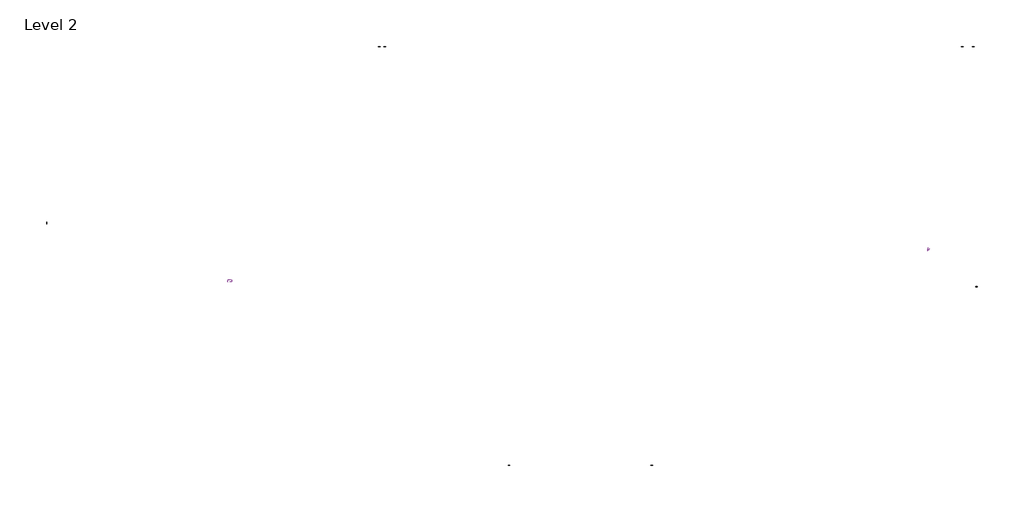
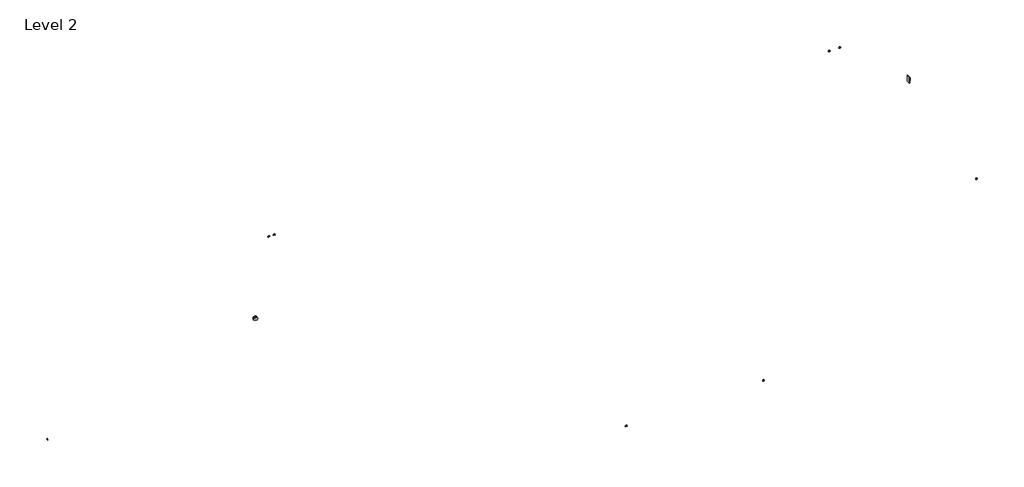
# One storey: 10 proxies.
"""IFC4 building model written with IfcOpenShell, lengths in millimetres."""

import ifcopenshell
import ifcopenshell.guid

model = None  # the IFC model being written
_history = None  # IfcOwnerHistory: only IFC2X3 demands one
_inside = {}  # id of a spatial element -> (the spatial element, [elements in it])
_under = {}  # id of a project, library or spatial element -> (it, [spatial elements below it])
_declared = {}  # id of a project -> (the project, [libraries it declares])
_typed = {}  # id of a type object -> (the type object, [elements of that type])
_made_of = {}  # id of a material, layer set ... -> (it, [elements and type objects made of it])


def new_model(schema):
    """Start an empty IFC model of exactly this schema.

    Asked for "IFC4X3", IfcOpenShell would pick the latest addendum, in which some entities
    have other attributes; the version numbers below select the first issue.
    IFC2X3 requires an IfcOwnerHistory on every rooted entity: one is made here for all.
    """
    global model, _history
    if schema == "IFC4X3":
        model = ifcopenshell.file(schema_version=(4, 3, 0, 0))
    else:
        model = ifcopenshell.file(schema=schema)
    _inside.clear()
    _under.clear()
    _declared.clear()
    _typed.clear()
    _made_of.clear()
    _history = None
    if model.schema == "IFC2X3":
        org = make("IfcOrganization", Name="unknown")
        user = make(
            "IfcPersonAndOrganization",
            ThePerson=make("IfcPerson", FamilyName="unknown"),
            TheOrganization=org,
        )
        app = make(
            "IfcApplication",
            ApplicationDeveloper=org,
            Version="unknown",
            ApplicationFullName="unknown",
            ApplicationIdentifier="unknown",
        )
        _history = make(
            "IfcOwnerHistory",
            OwningUser=user,
            OwningApplication=app,
            ChangeAction="ADDED",
            CreationDate=0,
        )
    return model


def make(cls, **values):
    """One entity of the class cls with the attributes given. An attribute that is None is left unset."""
    return model.create_entity(
        cls, **{name: value for name, value in values.items() if value is not None}
    )


def rooted(cls, **values):
    """An entity with a GlobalId (a new one), such as an element, a storey or a relation."""
    return make(cls, GlobalId=ifcopenshell.guid.new(), OwnerHistory=_history, **values)


def si_unit(unit_type, name, prefix=None):
    """IfcSIUnit, for example si_unit("LENGTHUNIT", "METRE", prefix="MILLI")."""
    return make("IfcSIUnit", UnitType=unit_type, Prefix=prefix, Name=name)


def assignment(units):
    """IfcUnitAssignment: the units of a project."""
    return None if units is None else make("IfcUnitAssignment", Units=units)


def point(xyz):
    """IfcCartesianPoint."""
    return None if xyz is None else make("IfcCartesianPoint", Coordinates=xyz)


def direction(xyz):
    """IfcDirection."""
    return None if xyz is None else make("IfcDirection", DirectionRatios=xyz)


def frame(location, z_axis=None, x_axis=None):
    """IfcAxis2Placement3D, a coordinate frame: its origin and axes. An axis left out is left unset."""
    return make(
        "IfcAxis2Placement3D",
        Location=point(location),
        Axis=direction(z_axis),
        RefDirection=direction(x_axis),
    )


def frame_2d(location, x_axis=None):
    """IfcAxis2Placement2D, a coordinate frame in the plane: its origin and x axis."""
    return make(
        "IfcAxis2Placement2D", Location=point(location), RefDirection=direction(x_axis)
    )


def origin():
    """The frame at (0, 0, 0) with its axes left unset."""
    return frame((0.0, 0.0, 0.0))


def origin_with_axes():
    """The frame at (0, 0, 0) with the z axis (0, 0, 1) and the x axis (1, 0, 0) written out."""
    return frame((0.0, 0.0, 0.0), z_axis=(0.0, 0.0, 1.0), x_axis=(1.0, 0.0, 0.0))


def origin_2d():
    """The frame at (0, 0) in the plane with its x axis left unset."""
    return frame_2d((0.0, 0.0))


def place(relative_to, where):
    """IfcLocalPlacement: puts the frame where relative to a parent placement (None: the world)."""
    return make(
        "IfcLocalPlacement", PlacementRelTo=relative_to, RelativePlacement=where
    )


def context(
    kind, dimensions, precision=None, world=None, true_north=None, identifier=None
):
    """IfcGeometricRepresentationContext, for example the 3D "Model" context."""
    return make(
        "IfcGeometricRepresentationContext",
        ContextIdentifier=identifier,
        ContextType=kind,
        CoordinateSpaceDimension=dimensions,
        Precision=precision,
        WorldCoordinateSystem=world,
        TrueNorth=true_north,
    )


def project(units=None, contexts=None):
    """IfcProject with its units and contexts."""
    return rooted(
        "IfcProject",
        Name="project",
        RepresentationContexts=contexts,
        UnitsInContext=assignment(units),
    )


def spatial(cls, under=None, at=None, **own):
    """A site, building, storey or space (cls), placed at a placement, below another one or the project."""
    s = rooted(cls, ObjectPlacement=at, **own)
    if under is not None:
        _under.setdefault(under.id(), (under, []))[1].append(s)
    return s


def polyline(points):
    """IfcPolyline through the points."""
    return make("IfcPolyline", Points=[point(p) for p in points])


def circle_curve(where, radius):
    """IfcCircle in the frame where."""
    return make("IfcCircle", Position=where, Radius=radius)


def ellipse_curve(where, semi_axis1, semi_axis2):
    """IfcEllipse in the frame where."""
    return make(
        "IfcEllipse", Position=where, SemiAxis1=semi_axis1, SemiAxis2=semi_axis2
    )


def trimmed(basis, trim1, trim2, sense, master):
    """IfcTrimmedCurve: the piece of a basis curve between two trims."""
    return make(
        "IfcTrimmedCurve",
        BasisCurve=basis,
        Trim1=trim1,
        Trim2=trim2,
        SenseAgreement=sense,
        MasterRepresentation=master,
    )


def segment(curve, same_sense, transition):
    """IfcCompositeCurveSegment."""
    return make(
        "IfcCompositeCurveSegment",
        Transition=transition,
        SameSense=same_sense,
        ParentCurve=curve,
    )


def composite_curve(segments, self_intersect=None):
    """IfcCompositeCurve: segments joined end to end."""
    return make("IfcCompositeCurve", Segments=segments, SelfIntersect=self_intersect)


def outline(outer, holes=None, kind="AREA"):
    """IfcArbitraryClosedProfileDef: a profile drawn as a closed curve; with holes, ...WithVoids."""
    if holes is None:
        return make("IfcArbitraryClosedProfileDef", ProfileType=kind, OuterCurve=outer)
    return make(
        "IfcArbitraryProfileDefWithVoids",
        ProfileType=kind,
        OuterCurve=outer,
        InnerCurves=holes,
    )


def extrude(swept, where, along, depth):
    """IfcExtrudedAreaSolid: the profile swept, set in the frame where, extruded along a direction by depth."""
    return make(
        "IfcExtrudedAreaSolid",
        SweptArea=swept,
        Position=where,
        ExtrudedDirection=direction(along),
        Depth=depth,
    )


def shape(context_of_items, identifier, shape_type, items):
    """IfcShapeRepresentation: the items that make up one representation, for example the "Body"."""
    return make(
        "IfcShapeRepresentation",
        ContextOfItems=context_of_items,
        RepresentationIdentifier=identifier,
        RepresentationType=shape_type,
        Items=items,
    )


def source(mapping_origin, context_of_items, identifier, shape_type, items):
    """IfcRepresentationMap: a shape defined once, which mapped items show again and again."""
    return make(
        "IfcRepresentationMap",
        MappingOrigin=mapping_origin,
        MappedRepresentation=shape(context_of_items, identifier, shape_type, items),
    )


def transform(
    local_origin,
    x_axis=None,
    y_axis=None,
    z_axis=None,
    scale=None,
    scale2=None,
    scale3=None,
    uniform=True,
):
    """IfcCartesianTransformationOperator3D, or its non-uniform kind. x_axis, y_axis, z_axis: its Axis1, 2, 3."""
    if uniform:
        return make(
            "IfcCartesianTransformationOperator3D",
            Axis1=direction(x_axis),
            Axis2=direction(y_axis),
            LocalOrigin=point(local_origin),
            Scale=scale,
            Axis3=direction(z_axis),
        )
    return make(
        "IfcCartesianTransformationOperator3DnonUniform",
        Axis1=direction(x_axis),
        Axis2=direction(y_axis),
        LocalOrigin=point(local_origin),
        Scale=scale,
        Axis3=direction(z_axis),
        Scale2=scale2,
        Scale3=scale3,
    )


def mapped(mapping_source, mapping_target):
    """IfcMappedItem: shows the shape of a source again, moved by a transform."""
    return make(
        "IfcMappedItem", MappingSource=mapping_source, MappingTarget=mapping_target
    )


def made_of(thing, what):
    """Note that an element or type object is made of a material, layer set ...; save() writes the relation."""
    if what is not None:
        _made_of.setdefault(what.id(), (what, []))[1].append(thing)
    return thing


def element(
    cls,
    number,
    at=None,
    inside=None,
    cuts=None,
    type_object=None,
    material=None,
    context=None,
    identifier="Body",
    shape_type=None,
    held_by="IfcProductDefinitionShape",
    body=None,
    shapes=None,
    **own,
):
    """One element of the class cls, such as IfcWall. Its Tag is "e" and its number.

    at: its placement. inside: the storey or other place that contains it. cuts: it is an
    opening in that element (IfcRelVoidsElement). A single representation is given by context,
    identifier, shape_type and body (its items); several are given by shapes. held_by: the class
    of the entity that holds the representations. save() writes the other relations.
    """
    e = rooted(cls, Tag="e%d" % number, ObjectPlacement=at, **own)
    if body is not None:
        shapes = [shape(context, identifier, shape_type, body)]
    if shapes is not None:
        e.Representation = make(held_by, Representations=shapes)
    if inside is not None:
        _inside.setdefault(inside.id(), (inside, []))[1].append(e)
    if cuts is not None:
        rooted(
            "IfcRelVoidsElement", RelatingBuildingElement=cuts, RelatedOpeningElement=e
        )
    if type_object is not None:
        _typed.setdefault(type_object.id(), (type_object, []))[1].append(e)
    return made_of(e, material)


def aggregate(whole, parts):
    """IfcRelAggregates: a whole, such as a stair, and the parts it consists of."""
    return rooted("IfcRelAggregates", RelatingObject=whole, RelatedObjects=parts)


def save(model, path):
    """Write the relations noted so far, then the file.

    IfcRelAggregates (storeys below a building ...), IfcRelContainedInSpatialStructure (elements
    in a storey), IfcRelDefinesByType, IfcRelAssociatesMaterial and IfcRelDeclares: one each for
    every whole, place, type object, material and project.
    """
    for whole, parts in _under.values():
        aggregate(whole, parts)
    for where, things in _inside.values():
        rooted(
            "IfcRelContainedInSpatialStructure",
            RelatedElements=things,
            RelatingStructure=where,
        )
    for kind, things in _typed.values():
        rooted("IfcRelDefinesByType", RelatedObjects=things, RelatingType=kind)
    for what, things in _made_of.values():
        rooted("IfcRelAssociatesMaterial", RelatedObjects=things, RelatingMaterial=what)
    for by, libraries in _declared.values():
        rooted("IfcRelDeclares", RelatingContext=by, RelatedDefinitions=libraries)
    model.write(path)


def plane_surface(at):
    """IfcPlane: the flat surface through the origin of the frame at, square to its z axis."""
    return make("IfcPlane", Position=at)


def cylinder_surface(at, radius):
    """IfcCylindricalSurface: all points at the distance radius from the z axis of the frame at."""
    return make("IfcCylindricalSurface", Position=at, Radius=radius)


def revolved_surface(curve, axis_point, axis_direction):
    """IfcSurfaceOfRevolution: the curve turned about the line through axis_point along axis_direction."""
    return make(
        "IfcSurfaceOfRevolution",
        SweptCurve=make("IfcArbitraryOpenProfileDef", ProfileType="CURVE", Curve=curve),
        AxisPosition=make("IfcAxis1Placement", Location=point(axis_point), Axis=direction(axis_direction)),
    )


def advanced_brep(points, edges, surfaces, faces):
    """IfcAdvancedBrep: a solid bounded by faces that lie on surfaces and meet in shared edges.

    An edge is (start, end): straight between two places in points (the first is 0);
    or (start, end, curve); or (start, end, curve, False) where it runs against its curve.
    A face is (place in surfaces, loops), or (place, loops, False) where it looks against
    its surface's normal. A loop lists edges by number (the first is 1), with a minus sign
    where the edge is run from its end to its start. The first loop is the outer one.
    """
    corners = [point(p) for p in points]
    vertices = [make("IfcVertexPoint", VertexGeometry=c) for c in corners]
    made = []
    for start, end, *more in edges:
        made.append(
            make(
                "IfcEdgeCurve",
                EdgeStart=vertices[start],
                EdgeEnd=vertices[end],
                EdgeGeometry=more[0] if more else make("IfcPolyline", Points=[corners[start], corners[end]]),
                SameSense=more[1] if len(more) > 1 else True,
            )
        )
    hull = []
    for where, loops, *sense in faces:
        bounds = []
        for j, loop in enumerate(loops):
            ring = [make("IfcOrientedEdge", EdgeElement=made[abs(k) - 1], Orientation=k > 0) for k in loop]
            bounds.append(
                make(
                    "IfcFaceOuterBound" if j == 0 else "IfcFaceBound",
                    Bound=make("IfcEdgeLoop", EdgeList=ring),
                    Orientation=True,
                )
            )
        hull.append(make("IfcAdvancedFace", Bounds=bounds, FaceSurface=surfaces[where], SameSense=sense[0] if sense else True))
    return make("IfcAdvancedBrep", Outer=make("IfcClosedShell", CfsFaces=hull))


def magnetic_contact_standard_5e95dac8(model_context):
    return source(origin(), model_context, "Body", "SweptSolid", [
        extrude(outline(polyline([(32.0, -13.0), (-32.0, -13.0), (-32.0, 0.0), (32.0, 0.0), (32.0, -13.0)])), frame((0.0, 0.0, 15.5767529), z_axis=(0.0, 0.0, 1.0), x_axis=(1.0, 0.0, 0.0)), (0.0, 0.0, 1.0), 9.4232471),
        extrude(outline(polyline([(32.0, -13.0), (-32.0, -13.0), (-32.0, 0.0), (32.0, 0.0), (32.0, -13.0)])), origin_with_axes(), (0.0, 0.0, 1.0), 8.0),
        extrude(outline(polyline([(19.5, -13.0), (-19.5, -13.0), (-19.5, 0.0), (19.5, 0.0), (19.5, -13.0)])), frame((0.0, 0.0, -20.0), z_axis=(0.0, 0.0, 1.0), x_axis=(1.0, 0.0, 0.0)), (0.0, 0.0, 1.0), 20.0),
    ])


def magnetic_contact_standard_a188dc91(model_context):
    return source(origin(), model_context, "Body", "SweptSolid", [
        extrude(outline(polyline([(32.0, 13.0), (32.0, 0.0), (-32.0, 0.0), (-32.0, 13.0), (32.0, 13.0)])), frame((0.0, 0.0, 15.5767529), z_axis=(0.0, 0.0, 1.0), x_axis=(1.0, 0.0, 0.0)), (0.0, 0.0, 1.0), 9.4232471),
        extrude(outline(polyline([(32.0, 13.0), (32.0, 0.0), (-32.0, 0.0), (-32.0, 13.0), (32.0, 13.0)])), origin_with_axes(), (0.0, 0.0, 1.0), 8.0),
        extrude(outline(polyline([(19.5, 13.0), (19.5, 0.0), (-19.5, 0.0), (-19.5, 13.0), (19.5, 13.0)])), frame((0.0, 0.0, -20.0), z_axis=(0.0, 0.0, 1.0), x_axis=(1.0, 0.0, 0.0)), (0.0, 0.0, 1.0), 20.0),
    ])


def standard_da8f596e(model_context):
    return source(origin(), model_context, "Body", "SolidModel", [
        extrude(outline(polyline([(-50.8099209, -85.0), (-52.6934767, -85.0), (-52.6934767, -80.0), (-50.8099209, -80.0), (-50.8099209, -85.0)])), frame((0.0, 0.0, 4.6605901), z_axis=(0.0, 0.0, 1.0), x_axis=(1.0, 0.0, 0.0)), (0.0, 0.0, 1.0), 15.0684465),
        extrude(outline(polyline([(4.6605901, -47.0428093), (4.6605901, -45.1592535), (16.6020397, -45.1592535), (4.6605901, -37.2865788), (4.6605901, -35.2705855), (19.7290366, -35.2705855), (19.7290366, -37.1541413), (7.7912659, -37.1541413), (19.7290366, -45.026816), (19.7290366, -47.0428093), (4.6605901, -47.0428093)])), frame((0.0, -85.0, 0.0), z_axis=(0.0, 1.0, 0.0), x_axis=(0.0, 0.0, 1.0)), (0.0, 0.0, 1.0), 5.0),
        extrude(outline(polyline([(4.6605901, -28.2072512), (4.6605901, -26.3236953), (17.8454808, -26.3236953), (17.8454808, -21.3793613), (19.7290366, -21.3793613), (19.7290366, -33.1515852), (17.8454808, -33.1515852), (17.8454808, -28.2072512), (4.6605901, -28.2072512)])), frame((0.0, -85.0, 0.0), z_axis=(0.0, 1.0, 0.0), x_axis=(0.0, 0.0, 1.0)), (0.0, 0.0, 1.0), 5.0),
        extrude(outline(polyline([(4.6605901, -19.260361), (4.6605901, -17.3768052), (11.2530355, -17.3768052), (9.8514051, -12.1197715), (7.7839082, -10.7034258), (4.6605901, -8.7426148), (4.6605901, -6.5537169), (8.7440802, -9.0663509), (11.4884799, -11.6635978), (12.8901103, -8.5090097), (15.6050795, -7.4881372), (17.8841084, -8.1043395), (19.322527, -9.7524509), (19.7290366, -12.7672438), (19.7290366, -19.260361), (4.6605901, -19.260361)]), holes=[polyline([(13.1365913, -17.3768052), (17.8454808, -17.3768052), (17.8454808, -12.6863098), (17.1943297, -10.1681575), (13.4033057, -11.0106073), (13.1365913, -13.1608775), (13.1365913, -17.3768052)])]), frame((0.0, -85.0, 0.0), z_axis=(0.0, 1.0, 0.0), x_axis=(0.0, 0.0, 1.0)), (0.0, 0.0, 1.0), 5.0),
        extrude(outline(polyline([(19.7290366, 5.6967535), (11.1022038, 5.6967535), (7.298304, 4.7439392), (6.3087014, 1.5544023), (6.809021, -0.6602474), (8.2308849, -1.9367979), (11.1022038, -2.3083587), (19.7290366, -2.3083587), (19.7290366, -4.1919145), (11.0359851, -4.1919145), (7.2633552, -3.619858), (5.153552, -1.7105504), (4.4251456, 1.7309856), (5.2620772, 5.2258646), (7.4325809, 7.0689534), (11.0359851, 7.5803093), (19.7290366, 7.5803093), (19.7290366, 5.6967535)])), frame((0.0, -85.0, 0.0), z_axis=(0.0, 1.0, 0.0), x_axis=(0.0, 0.0, 1.0)), (0.0, 0.0, 1.0), 5.0),
        extrude(outline(polyline([(4.6605901, 10.876532), (4.6605901, 16.3248644), (4.9181075, 18.7473673), (5.674105, 20.5481497), (7.0407866, 21.9240283), (9.2352027, 22.9540979), (12.2757474, 23.3550893), (15.858918, 22.7627993), (18.434092, 20.9785716), (19.5119862, 18.763922), (19.7290366, 16.0747046), (19.7290366, 10.876532), (4.6605901, 10.876532)]), holes=[polyline([(6.5441459, 12.7600878), (17.8454808, 12.7600878), (17.8454808, 16.0415952), (17.5438176, 18.7124185), (15.8736333, 20.6677113), (12.305178, 21.4715335), (9.4559319, 21.0613451), (7.585252, 19.9153926), (6.8163786, 18.5174411), (6.5441459, 16.0930987), (6.5441459, 12.7600878)])]), frame((0.0, -85.0, 0.0), z_axis=(0.0, 1.0, 0.0), x_axis=(0.0, 0.0, 1.0)), (0.0, 0.0, 1.0), 5.0),
        extrude(outline(polyline([(4.6605901, 25.9449785), (4.6605901, 37.010869), (6.5441459, 37.010869), (6.5441459, 27.8285344), (11.4884799, 27.8285344), (11.4884799, 36.3045355), (13.3720357, 36.3045355), (13.3720357, 27.8285344), (17.8454808, 27.8285344), (17.8454808, 36.7754245), (19.7290366, 36.7754245), (19.7290366, 25.9449785), (4.6605901, 25.9449785)])), frame((0.0, -85.0, 0.0), z_axis=(0.0, 1.0, 0.0), x_axis=(0.0, 0.0, 1.0)), (0.0, 0.0, 1.0), 5.0),
        extrude(outline(polyline([(4.6605901, 39.8362027), (4.6605901, 41.7197585), (11.2530355, 41.7197585), (9.8514051, 46.9767922), (7.7839082, 48.3931379), (4.6605901, 50.3539489), (4.6605901, 52.5428468), (8.7440802, 50.0302128), (11.4884799, 47.4329659), (12.8901103, 50.587554), (15.6050795, 51.6084265), (17.8841084, 50.9922242), (19.322527, 49.3441128), (19.7290366, 46.3293199), (19.7290366, 39.8362027), (4.6605901, 39.8362027)]), holes=[polyline([(13.1365913, 41.7197585), (17.8454808, 41.7197585), (17.8454808, 46.4102539), (17.1943297, 48.9284062), (13.4033057, 48.0859564), (13.1365913, 45.9356862), (13.1365913, 41.7197585)])]), frame((0.0, -85.0, 0.0), z_axis=(0.0, 1.0, 0.0), x_axis=(0.0, 0.0, 1.0)), (0.0, 0.0, 1.0), 5.0),
        extrude(outline(polyline([(-8.4558541, -53.6352547), (-11.3326913, -52.8222354), (-13.23832, -50.6940381), (-13.8710771, -47.3297573), (-13.2843053, -44.4805112), (-11.6398728, -42.5380943), (-9.3865955, -41.8630308), (-7.2565588, -42.4498026), (-5.7298485, -44.2726579), (-4.7843918, -47.6056688), (-2.4262682, -51.2808099), (-0.8627697, -50.4346813), (-0.2152974, -47.7381063), (-0.8701273, -45.0488889), (-2.8051866, -43.9820311), (-2.8051866, -42.0984753), (-0.447063, -42.8452757), (1.1311507, -44.8318385), (1.6682584, -47.8116827), (1.155063, -50.603907), (-0.3495743, -52.5113752), (-2.4814505, -53.1643657), (-4.3539698, -52.636455), (-5.7556002, -51.034329), (-6.6845023, -48.0820759), (-11.6435516, -45.435165), (-11.9875212, -47.4033337), (-11.533187, -49.6621291), (-10.3412493, -51.1446935), (-8.4558541, -51.7516988), (-8.4558541, -53.6352547)])), frame((0.0, -85.0, 0.0), z_axis=(0.0, 1.0, 0.0), x_axis=(0.0, 0.0, 1.0)), (0.0, 0.0, 1.0), 5.0),
        extrude(outline(polyline([(-13.6356326, -39.0376971), (-13.6356326, -27.9718067), (-11.7520768, -27.9718067), (-11.7520768, -37.1541413), (-6.8077427, -37.1541413), (-6.8077427, -28.6781401), (-4.9241869, -28.6781401), (-4.9241869, -37.1541413), (-0.4507419, -37.1541413), (-0.4507419, -28.2072512), (1.4328139, -28.2072512), (1.4328139, -39.0376971), (-13.6356326, -39.0376971)])), frame((0.0, -85.0, 0.0), z_axis=(0.0, 1.0, 0.0), x_axis=(0.0, 0.0, 1.0)), (0.0, 0.0, 1.0), 5.0),
        extrude(outline(polyline([(-8.2792707, -14.5514715), (-11.053101, -16.1499188), (-11.9875212, -19.0322742), (-11.3014213, -21.6313605), (-9.2284063, -23.4008729), (-5.9836871, -23.9692506), (-3.1841051, -23.4891646), (-1.020959, -21.8244985), (-0.2152974, -18.8777638), (-0.9418643, -16.3320203), (-3.2576815, -14.786916), (-2.8088655, -12.9033602), (0.4947149, -15.0315575), (1.6682584, -18.8041874), (0.7614293, -22.4241462), (-1.8928393, -24.9606925), (-5.9873659, -25.8528064), (-10.0156737, -25.0636995), (-12.8814745, -22.764437), (-13.8710771, -18.8446544), (-12.5632566, -14.9009594), (-8.764875, -12.6679157), (-8.2792707, -14.5514715)])), frame((0.0, -85.0, 0.0), z_axis=(0.0, 1.0, 0.0), x_axis=(0.0, 0.0, 1.0)), (0.0, 0.0, 1.0), 5.0),
        extrude(outline(polyline([(1.4328139, -0.1893584), (-7.1940188, -0.1893584), (-10.9979187, -1.1421728), (-11.9875212, -4.3317097), (-11.4872017, -6.5463593), (-10.0653378, -7.8229098), (-7.1940188, -8.1944706), (1.4328139, -8.1944706), (1.4328139, -10.0780264), (-7.2602376, -10.0780264), (-11.0328675, -9.5059699), (-13.1426707, -7.5966624), (-13.8710771, -4.1551263), (-13.0341455, -0.6602474), (-10.8636417, 1.1828414), (-7.2602376, 1.6941974), (1.4328139, 1.6941974), (1.4328139, -0.1893584)])), frame((0.0, -85.0, 0.0), z_axis=(0.0, 1.0, 0.0), x_axis=(0.0, 0.0, 1.0)), (0.0, 0.0, 1.0), 5.0),
        extrude(outline(polyline([(-13.6356326, 4.9904201), (-13.6356326, 6.8739759), (-7.0431872, 6.8739759), (-8.4448176, 12.1310096), (-10.5123144, 13.5473553), (-13.6356326, 15.5081663), (-13.6356326, 17.6970642), (-9.5521424, 15.1844302), (-6.8077427, 12.5871833), (-5.4061123, 15.7417714), (-2.6911432, 16.7626439), (-0.4121143, 16.1464416), (1.0263043, 14.4983303), (1.4328139, 11.4835373), (1.4328139, 4.9904201), (-13.6356326, 4.9904201)]), holes=[polyline([(-5.1596314, 6.8739759), (-0.4507419, 6.8739759), (-0.4507419, 11.5644713), (-1.101893, 14.0826236), (-4.892917, 13.2401738), (-5.1596314, 11.0899036), (-5.1596314, 6.8739759)])]), frame((0.0, -85.0, 0.0), z_axis=(0.0, 1.0, 0.0), x_axis=(0.0, 0.0, 1.0)), (0.0, 0.0, 1.0), 5.0),
        extrude(outline(polyline([(22.1778669, -85.0), (20.2943111, -85.0), (20.2943111, -80.0), (22.1778669, -80.0), (22.1778669, -85.0)])), frame((0.0, 0.0, -13.6356326), z_axis=(0.0, 0.0, 1.0), x_axis=(1.0, 0.0, 0.0)), (0.0, 0.0, 1.0), 15.0684465),
        extrude(outline(polyline([(-13.6356326, 29.7120902), (-13.6356326, 31.595646), (-0.4507419, 31.595646), (-0.4507419, 36.53998), (1.4328139, 36.53998), (1.4328139, 24.7677562), (-0.4507419, 24.7677562), (-0.4507419, 29.7120902), (-13.6356326, 29.7120902)])), frame((0.0, -85.0, 0.0), z_axis=(0.0, 1.0, 0.0), x_axis=(0.0, 0.0, 1.0)), (0.0, 0.0, 1.0), 5.0),
        extrude(outline(polyline([(-13.6356326, 42.8969809), (-13.6356326, 44.7805367), (-7.25288, 44.7805367), (1.4328139, 50.6666486), (1.4328139, 48.4446414), (-3.0369523, 45.5935559), (-5.5716592, 43.9822328), (-3.206178, 42.3745884), (1.4328139, 39.2328762), (1.4328139, 37.010869), (-7.25288, 42.8969809), (-13.6356326, 42.8969809)])), frame((0.0, -85.0, 0.0), z_axis=(0.0, 1.0, 0.0), x_axis=(0.0, 0.0, 1.0)), (0.0, 0.0, 1.0), 5.0),
        extrude(outline(polyline([(-31.9318553, -36.5544936), (-31.9318553, -34.564252), (-27.2229657, -32.8425643), (-27.2229657, -26.636395), (-31.9318553, -24.9110285), (-31.9318553, -22.9207869), (-16.8634087, -28.9356575), (-16.8634087, -30.539623), (-31.9318553, -36.5544936)]), holes=[polyline([(-25.3394099, -32.1509461), (-21.3111021, -30.6757393), (-18.7469645, -29.7376403), (-21.6348382, -28.6818189), (-25.3394099, -27.3243344), (-25.3394099, -32.1509461)])]), frame((0.0, -85.0, 0.0), z_axis=(0.0, 1.0, 0.0), x_axis=(0.0, 0.0, 1.0)), (0.0, 0.0, 1.0), 5.0),
        extrude(outline(polyline([(-31.9318553, -20.9084724), (-31.9318553, -11.4906933), (-30.0482994, -11.4906933), (-30.0482994, -19.0249166), (-16.8634087, -19.0249166), (-16.8634087, -20.9084724), (-31.9318553, -20.9084724)])), frame((0.0, -85.0, 0.0), z_axis=(0.0, 1.0, 0.0), x_axis=(0.0, 0.0, 1.0)), (0.0, 0.0, 1.0), 5.0),
        extrude(outline(polyline([(-31.9318553, -11.1264901), (-31.9318553, -9.1362485), (-27.2229657, -7.4145608), (-27.2229657, -1.2083915), (-31.9318553, 0.516975), (-31.9318553, 2.5072166), (-16.8634087, -3.507654), (-16.8634087, -5.1116195), (-31.9318553, -11.1264901)]), holes=[polyline([(-25.3394099, -6.7229426), (-21.3111021, -5.2477358), (-18.7469645, -4.3096367), (-21.6348382, -3.2538154), (-25.3394099, -1.8963309), (-25.3394099, -6.7229426)])]), frame((0.0, -85.0, 0.0), z_axis=(0.0, 1.0, 0.0), x_axis=(0.0, 0.0, 1.0)), (0.0, 0.0, 1.0), 5.0),
        extrude(outline(polyline([(-31.9318553, 4.5195311), (-31.9318553, 6.403087), (-25.3394099, 6.403087), (-26.7410403, 11.6601207), (-28.8085371, 13.0764663), (-31.9318553, 15.0372774), (-31.9318553, 17.2261753), (-27.8483651, 14.7135412), (-25.1039654, 12.1162943), (-23.702335, 15.2708824), (-20.9873659, 16.291755), (-18.7083369, 15.6755526), (-17.2699183, 14.0274413), (-16.8634087, 11.0126484), (-16.8634087, 4.5195311), (-31.9318553, 4.5195311)]), holes=[polyline([(-23.4558541, 6.403087), (-18.7469645, 6.403087), (-18.7469645, 11.0935824), (-19.3981157, 13.6117347), (-23.1891396, 12.7692849), (-23.4558541, 10.6190146), (-23.4558541, 6.403087)])]), frame((0.0, -85.0, 0.0), z_axis=(0.0, 1.0, 0.0), x_axis=(0.0, 0.0, 1.0)), (0.0, 0.0, 1.0), 5.0),
        extrude(outline(polyline([(-31.9318553, 19.5879777), (-31.9318553, 21.4715335), (-18.7469645, 21.4715335), (-31.9318553, 25.2570392), (-31.9318553, 27.8101403), (-18.7469645, 31.595646), (-31.9318553, 31.595646), (-31.9318553, 33.4792018), (-16.8634087, 33.4792018), (-16.8634087, 30.2381614), (-27.3002209, 27.2068138), (-29.7024904, 26.5335897), (-27.4841619, 25.9118692), (-16.8634087, 22.829018), (-16.8634087, 19.5879777), (-31.9318553, 19.5879777)])), frame((0.0, -85.0, 0.0), z_axis=(0.0, 1.0, 0.0), x_axis=(0.0, 0.0, 1.0)), (0.0, 0.0, 1.0), 5.0),
        extrude(outline(composite_curve([segment(polyline([(38.0, 64.6606526), (38.0, -64.6606526)]), True, "CONTINUOUS"), segment(trimmed(circle_curve(origin_2d(), 75.0), [point((38.0, -64.6606526))], [point((0.0, -75.0))], False, "CARTESIAN"), True, "CONTINUOUS"), segment(trimmed(circle_curve(origin_2d(), 75.0), [point((0.0, -75.0))], [point((-56.0, -49.8898787))], False, "CARTESIAN"), True, "CONTINUOUS"), segment(polyline([(-56.0, -49.8898787), (-56.0, 49.8898787)]), True, "CONTINUOUS"), segment(trimmed(circle_curve(origin_2d(), 75.0), [point((-56.0, 49.8898787))], [point((0.0, 75.0))], False, "CARTESIAN"), True, "CONTINUOUS"), segment(trimmed(circle_curve(origin_2d(), 75.0), [point((0.0, 75.0))], [point((38.0, 64.6606526))], False, "CARTESIAN"), True, "CONTINUOUS")], self_intersect=False)), frame((0.0, -30.0, 0.0), z_axis=(0.0, 1.0, 0.0), x_axis=(0.0, 0.0, 1.0)), (0.0, 0.0, 1.0), 30.0),
        advanced_brep(
        [(-65.0, -80.0, 0.0), (65.0, -80.0, 0.0), (0.0, -80.0, 0.0), (-75.0, -70.0, 0.0), (75.0, -70.0, 0.0), (-75.0, -30.0, 0.0), (75.0, -30.0, 0.0), (0.0, -30.0, 0.0)],
        [
            (0, 1, circle_curve(frame((0.0, -80.0, 0.0), z_axis=(0.0, -1.0, 0.0), x_axis=(1.0, 0.0, 0.0)), 65.0)),
            (1, 2),
            (2, 0),
            (1, 0, circle_curve(frame((0.0, -80.0, 0.0), z_axis=(0.0, -1.0, 0.0), x_axis=(1.0, 0.0, 0.0)), 65.0)),
            (3, 4, circle_curve(frame((0.0, -70.0, 0.0), z_axis=(0.0, -1.0, 0.0), x_axis=(1.0, 0.0, 0.0)), 75.0)),
            (4, 1, circle_curve(frame((65.0, -70.0, 0.0), z_axis=(0.0, 0.0, -1.0), x_axis=(-1.0, 0.0, 0.0)), 10.0)),
            (0, 3, circle_curve(frame((-65.0, -70.0, 0.0), z_axis=(0.0, 0.0, -1.0), x_axis=(1.0, 0.0, 0.0)), 10.0)),
            (4, 3, circle_curve(frame((0.0, -70.0, 0.0), z_axis=(0.0, -1.0, 0.0), x_axis=(1.0, 0.0, 0.0)), 75.0)),
            (5, 6, circle_curve(frame((0.0, -30.0, 0.0), z_axis=(0.0, -1.0, 0.0), x_axis=(1.0, 0.0, 0.0)), 75.0)),
            (6, 4),
            (3, 5),
            (6, 5, circle_curve(frame((0.0, -30.0, 0.0), z_axis=(0.0, -1.0, 0.0), x_axis=(1.0, 0.0, 0.0)), 75.0)),
            (7, 6),
            (5, 7),
        ],
        [
            plane_surface(frame((0.0, -80.0, 0.0), z_axis=(0.0, -1.0, 0.0), x_axis=(1.0, 0.0, 0.0))),
            revolved_surface(trimmed(ellipse_curve(frame((65.0, -70.0, 0.0), z_axis=(0.0, 0.0, 1.0), x_axis=(-1.0, 0.0, 0.0)), 10.0, 10.0), [point((65.0, -80.0, 0.0))], [point((75.0, -70.0, 0.0))], True, "CARTESIAN"), (0.0, 0.0, 0.0), (0.0, 1.0, 0.0)),
            cylinder_surface(frame((0.0, 0.0, 0.0), z_axis=(0.0, 1.0, 0.0), x_axis=(1.0, 0.0, 0.0)), 75.0),
            plane_surface(frame((0.0, -30.0, 0.0), z_axis=(0.0, 1.0, 0.0), x_axis=(1.0, 0.0, 0.0))),
        ],
        [
            (0, [[1, 2, 3]]),
            (0, [[4, -3, -2]]),
            (1, [[5, 6, -1, 7]]),
            (1, [[8, -7, -4, -6]]),
            (2, [[9, 10, -5, 11]]),
            (2, [[12, -11, -8, -10]]),
            (3, [[13, -9, 14]]),
            (3, [[-14, -12, -13]]),
        ],
    ),
    ])


def wall_mounted_passive_infrared_detector_standard_722f1ccb(model_context):
    return source(origin(), model_context, "Body", "SweptSolid", [
        extrude(outline(polyline([(64.0, 0.0), (64.0, -234.0), (-64.0, -234.0), (-64.0, 0.0), (64.0, 0.0)])), origin_with_axes(), (0.0, 0.0, 1.0), 3.3125),
        extrude(outline(polyline([(32.0, -58.5), (32.0, -175.5), (-32.0, -175.5), (-32.0, -58.5), (32.0, -58.5)])), frame((0.0, 0.0, -53.0), z_axis=(0.0, 0.0, 1.0), x_axis=(1.0, 0.0, 0.0)), (0.0, 0.0, 1.0), 53.0),
    ])


model = new_model("IFC4")

# Units and contexts
model_context = context("Model", 3, world=origin())
ifc_project = project(units=[si_unit("LENGTHUNIT", "METRE", prefix="MILLI")], contexts=[model_context])

# Site, building, storey
site = spatial("IfcSite", under=ifc_project)
building = spatial("IfcBuilding", under=site)
storey = spatial("IfcBuildingStorey", under=building, Name="Level 2", Elevation=103800.0)

# Proxies
placement = place(None, origin())
magnetic_contact_standard_shape = magnetic_contact_standard_5e95dac8(model_context)
element("IfcBuildingElementProxy", 1, Name="Magnetic Contact : Standard", ObjectType="Magnetic Contact : Standard", at=placement, inside=storey, context=model_context, shape_type="MappedRepresentation", body=[
    mapped(magnetic_contact_standard_shape, transform((16896.6410372, -52.0, 102273.0), x_axis=(-1.0, 0.0, 0.0), y_axis=(0.0, 1.0, 0.0), z_axis=(0.0, 0.0, -1.0))),
])
element("IfcBuildingElementProxy", 2, Name="Magnetic Contact : Standard", ObjectType="Magnetic Contact : Standard", at=placement, inside=storey, context=model_context, shape_type="MappedRepresentation", body=[
    mapped(magnetic_contact_standard_shape, transform((22135.4766651, -52.0, 102273.0), x_axis=(-1.0, 0.0, 0.0), y_axis=(0.0, 1.0, 0.0), z_axis=(0.0, 0.0, -1.0))),
])
element("IfcBuildingElementProxy", 3, Name="Magnetic Contact : Standard", ObjectType="Magnetic Contact : Standard", at=placement, inside=storey, context=model_context, shape_type="MappedRepresentation", body=[
    mapped(magnetic_contact_standard_shape, transform((34045.091037, 6498.0, 102273.0), x_axis=(-1.0, 0.0, 0.0), y_axis=(0.0, 1.0, 0.0), z_axis=(0.0, 0.0, -1.0))),
])
element("IfcBuildingElementProxy", 4, Name="Magnetic Contact : Standard", ObjectType="Magnetic Contact : Standard", at=placement, inside=storey, context=model_context, shape_type="MappedRepresentation", body=[
    mapped(magnetic_contact_standard_shape, transform((-52.0, 8830.0730002, 102273.0), x_axis=(0.0, 1.0, 0.0), y_axis=(1.0, 0.0, 0.0), z_axis=(0.0, 0.0, -1.0))),
])
element("IfcBuildingElementProxy", 5, Name="Magnetic Contact : Standard", ObjectType="Magnetic Contact : Standard", at=placement, inside=storey, context=model_context, shape_type="MappedRepresentation", body=[
    mapped(magnetic_contact_standard_shape, transform((12135.564496, 15302.0, 102273.0), x_axis=(1.0, 0.0, 0.0), y_axis=(0.0, -1.0, 0.0), z_axis=(0.0, 0.0, -1.0))),
])
element("IfcBuildingElementProxy", 6, Name="Magnetic Contact : Standard", ObjectType="Magnetic Contact : Standard", at=placement, inside=storey, context=model_context, shape_type="MappedRepresentation", body=[
    mapped(magnetic_contact_standard_shape, transform((33521.1915602, 15302.0, 102273.0), x_axis=(1.0, 0.0, 0.0), y_axis=(0.0, -1.0, 0.0), z_axis=(0.0, 0.0, -1.0))),
])
element("IfcBuildingElementProxy", 7, Name="Magnetic Contact : Standard", ObjectType="Magnetic Contact : Standard", at=placement, inside=storey, context=model_context, shape_type="MappedRepresentation", body=[
    mapped(magnetic_contact_standard_shape, transform((33921.1915602, 15302.0, 102273.0), x_axis=(1.0, 0.0, 0.0), y_axis=(0.0, -1.0, 0.0), z_axis=(0.0, 0.0, -1.0))),
])
magnetic_contact_standard_2_shape = magnetic_contact_standard_a188dc91(model_context)
element("IfcBuildingElementProxy", 8, Name="Magnetic Contact : Standard", ObjectType="Magnetic Contact : Standard", at=placement, inside=storey, context=model_context, shape_type="MappedRepresentation", body=[
    mapped(magnetic_contact_standard_2_shape, transform((12341.4564448, 15302.0, 102273.0), x_axis=(-1.0, 0.0, 0.0), y_axis=(0.0, 1.0, 0.0), z_axis=(0.0, 0.0, -1.0))),
])
standard_shape = standard_da8f596e(model_context)
element("IfcBuildingElementProxy", 9, Name="Intruder Security Alarm Sounder : Standard", ObjectType="Intruder Security Alarm Sounder : Standard", at=placement, inside=storey, context=model_context, shape_type="MappedRepresentation", body=[
    mapped(standard_shape, transform((6650.0145244, 6670.0, 106100.0), x_axis=(-1.0, 0.0, 0.0), y_axis=(0.0, -1.0, 0.0), z_axis=(0.0, 0.0, 1.0))),
])
wall_mounted_passive_infrared_detector_standard_shape = wall_mounted_passive_infrared_detector_standard_722f1ccb(model_context)
element("IfcBuildingElementProxy", 10, Name="Wall Mounted Passive Infrared Detector : Standard", ObjectType="Wall Mounted Passive Infrared Detector : Standard", at=placement, inside=storey, context=model_context, shape_type="MappedRepresentation", body=[
    mapped(wall_mounted_passive_infrared_detector_standard_shape, transform((32250.0, 7873.3474956, 106200.0), x_axis=(0.0, -1.0, 0.0), y_axis=(0.0, 0.0, 1.0), z_axis=(-1.0, 0.0, 0.0))),
])

save(model, "model.ifc")

# Revit data of these elements
# Type "Magnetic Contact : Standard"
#   Type Mark = "Magnetic Contact"
#   Classification.OmniClass.23.Number = "23-29 11 21"
#   Classification.OmniClass.23.Description = "Security Sensors"
#   COBie.Type.CreatedBy = "info@mma.ie"
#   COBie.Type.CreatedOn = "2017-07-26T09:12:44"
#   COBie.Type.Name = "Magnetic Contact"
#   COBie.Type.Category = "23-29 11 21 : Security Sensors"
#   COBie.Type.Description = "Magnetic Contact_Standard"
#   COBie.Type.AssetType = "Fixed"
#   COBie.Type.Manufacturer = ""
#   COBie.Type.ModelNumber = ""
#   Keynote = "41 24 33.A"
#   COBie.Type.ReplacementCost = 0
#   MC_Width = 64 mm
#   MC_Height = 25 mm
#   MC_Depth = 13 mm
#   Default Elevation = 1200 mm
#   COBie.Type = yes
#   URL = ""
#   Model = ""
#   Manufacturer = ""
# Type "Intruder Security Alarm Sounder : Standard"
#   Type Mark = "Intruder Security Alarm Sounder"
#   Classification.OmniClass.21.Number = "21-04 70 50"
#   Classification.MasterFormat.Description = "Electronic Detection and Alarm"
#   Classification.OmniClass.21.Description = "Detection and Alarm"
#   Classification.UniFormat.II.Description = "Detection and Alarm"
#   Classification.MasterFormat.Number = "28 30 00"
#   Classification.OmniClass.23.Number = "23-29 11 23 15"
#   Classification.OmniClass.23.Description = "Intrusion Detection Microwave Alarms"
#   Classification.UniFormat.II.Number = "D7050"
#   COBie.Type.CreatedBy = "info@mma.ie"
#   COBie.Type.CreatedOn = "2017-07-26T09:25:07"
#   COBie.Type.Name = "Intruder Security Alarm Sounder"
#   COBie.Type.Category = "23-29 11 23 15 : Intrusion Detection Microwave Alarms"
#   COBie.Type.Description = "Intruder Security Alarm Sounder_Intruder Security Alarm Sounder"
#   COBie.Type.AssetType = "Fixed"
#   COBie.Type.Manufacturer = ""
#   COBie.Type.ModelNumber = ""
#   Standard = ""
#   SounderType = ""
#   SounderCutOffTimeMaximum = ""
#   PowerSupply = ""
#   Mounting = ""
#   Keynote = "28 01 30.51.A"
#   IntegralBeacon = ""
#   IngressProtectionStandard = ""
#   I.A. Audio Level = "75dB"
#   DirectionalOutputAt1MMinimum = ""
#   COBie.Type.ReplacementCost = 0
#   UsageCurrent = 0
#   SounderRadius = 75 mm
#   SounderDepth = 50 mm
#   PlanSymbolOffset [instance default] = 250 mm
#   PlanSymbolAlignment [instance default] = 0 mm
#   PhaseAngle = 0.00°
#   NominalVoltage = 0
#   NominalLength = 150 mm
#   NominalHeight = 80 mm
#   NominalFrequencyRange = 0
#   NominalCurrent = 0
#   I.A. Diameter = 150 mm
#   I.A. Depth = 50 mm
#   BaseLevelOffset = 0 mm
#   BackingCaseDepth = 30 mm
#   COBie.Type = yes
#   PlanSymbolVisibility [instance default] = yes
#   PlanObjectVisibility [instance default] = yes
#   NumberOfPoles = 0
#   HasProtectiveEarth = yes
#   URL = ""
#   Type Comments = ""
#   Model = ""
#   Manufacturer = ""
#   Description = (empty or 0)
#   Default Elevation = 0
#   Assembly Code = ""
# Type "Wall Mounted Passive Infrared Detector : Standard"
#   Type Mark = "Wall Mounted Passive Infrared Detector"
#   Classification.OmniClass.21.Number = "21-04 70 70 10"
#   Classification.OmniClass.21.Description = "Electronic Detention Monitoring and Control"
#   Classification.UniFormat.II.Description = "Intruction Detection"
#   Classification.OmniClass.23.Number = "23-29 11 21"
#   Classification.OmniClass.23.Description = "Security Sensors"
#   Classification.UniFormat.II.Number = "D7010.50"
#   COBie.Type.CreatedBy = "info@mma.ie"
#   COBie.Type.CreatedOn = "2017-07-26T09:12:44"
#   COBie.Type.Name = "Wall Mounted Passive Infrared Detector"
#   COBie.Type.Category = "23-29 11 21 : Security Sensors"
#   COBie.Type.Description = "Wall Mounted Passive Infrared Detector_Standard"
#   COBie.Type.AssetType = "Movable"
#   COBie.Type.Manufacturer = ""
#   COBie.Type.ModelNumber = ""
#   COBie.Type.ModelReference = ""
#   COBie.Type.Color = "White"
#   Units = "Volts"
#   Label = "PIR"
#   Keynote = "28 16 19.A"
#   COBie.Type.ReplacementCost = 0
#   Width 1 = 128 mm
#   Sensor Voltage = 230 V
#   PIR_Width = 64 mm
#   PIR_Depth = 53 mm
#   PIR Height = 117 mm
#   Length 1 = 234 mm
#   Height 1 = 3.312 mm
#   Default Elevation = 1200 mm
#   Sensor Width = 64 mm
#   Sensor Length = 117 mm
#   Sensor Height = 53 mm
#   Apparent Load = 0 VA
#   COBie.Type = yes
#   Sensor Number of Poles = 1
#   Sensor Material = none
#   Load Classification = Other
#   Cover Material = none
#   URL = ""
#   Model = ""
#   Manufacturer = ""
# Element 1 (IfcBuildingElementProxy, "Magnetic Contact : Standard")
#   Mark = "1"
#   COBie.CreatedBy = "info@mma.ie"
#   COBie.CreatedOn = "2017-07-26T09:12:43"
#   COBie.Component.Name = "Magnetic Contact-1"
#   COBie.Component.Space = "118"
#   COBie.Component.Description = "Magnetic Contact: Standard"
#   Notes = "n/a"
#   Color = "White"
#   Voltage = 12 V
#   Power = 3 W
#   COBie = yes
#   Phase Created = New Construction
# Element 2 (IfcBuildingElementProxy, "Magnetic Contact : Standard")
#   Mark = "2"
#   COBie.CreatedBy = "info@mma.ie"
#   COBie.CreatedOn = "2017-07-26T09:12:43"
#   COBie.Component.Name = "Magnetic Contact-2"
#   COBie.Component.Space = "118"
#   COBie.Component.Description = "Magnetic Contact: Standard"
#   Notes = "n/a"
#   Color = "White"
#   Voltage = 12 V
#   Power = 3 W
#   COBie = yes
#   Phase Created = New Construction
# Element 3 (IfcBuildingElementProxy, "Magnetic Contact : Standard")
#   Mark = "3"
#   COBie.CreatedBy = "info@mma.ie"
#   COBie.CreatedOn = "2017-07-26T09:12:43"
#   COBie.Component.Name = "Magnetic Contact-3"
#   COBie.Component.Space = "116"
#   COBie.Component.Description = "Magnetic Contact: Standard"
#   Notes = "n/a"
#   Color = "White"
#   Voltage = 12 V
#   Power = 3 W
#   COBie = yes
#   Phase Created = New Construction
# Element 4 (IfcBuildingElementProxy, "Magnetic Contact : Standard")
#   Mark = "4"
#   COBie.CreatedBy = "info@mma.ie"
#   COBie.CreatedOn = "2017-07-26T09:12:43"
#   COBie.Component.Name = "Magnetic Contact-4"
#   COBie.Component.Space = "101"
#   COBie.Component.Description = "Magnetic Contact: Standard"
#   Notes = "n/a"
#   Color = "White"
#   Voltage = 12 V
#   Power = 3 W
#   COBie = yes
#   Phase Created = New Construction
# Element 5 (IfcBuildingElementProxy, "Magnetic Contact : Standard")
#   Mark = "5"
#   COBie.CreatedBy = "info@mma.ie"
#   COBie.CreatedOn = "2017-07-26T09:12:43"
#   COBie.Component.Name = "Magnetic Contact-5"
#   COBie.Component.Space = "105"
#   COBie.Component.Description = "Magnetic Contact: Standard"
#   Notes = "n/a"
#   Color = "White"
#   Voltage = 12 V
#   Power = 3 W
#   COBie = yes
#   Phase Created = New Construction
# Element 6 (IfcBuildingElementProxy, "Magnetic Contact : Standard")
#   Mark = "7"
#   COBie.CreatedBy = "info@mma.ie"
#   COBie.CreatedOn = "2017-07-26T09:12:43"
#   COBie.Component.Name = "Magnetic Contact-7"
#   COBie.Component.Space = "115"
#   COBie.Component.Description = "Magnetic Contact: Standard"
#   Notes = "n/a"
#   Color = "White"
#   Voltage = 12 V
#   Power = 3 W
#   COBie = yes
#   Phase Created = New Construction
# Element 7 (IfcBuildingElementProxy, "Magnetic Contact : Standard")
#   Mark = "8"
#   COBie.CreatedBy = "info@mma.ie"
#   COBie.CreatedOn = "2017-07-26T09:12:43"
#   COBie.Component.Name = "Magnetic Contact-8"
#   COBie.Component.Space = "115"
#   COBie.Component.Description = "Magnetic Contact: Standard"
#   Notes = "n/a"
#   Color = "White"
#   Voltage = 12 V
#   Power = 3 W
#   COBie = yes
#   Phase Created = New Construction
# Element 8 (IfcBuildingElementProxy, "Magnetic Contact : Standard")
#   Mark = "6"
#   COBie.CreatedBy = "info@mma.ie"
#   COBie.CreatedOn = "2017-07-26T09:12:43"
#   COBie.Component.Name = "Magnetic Contact-6"
#   COBie.Component.Space = "105"
#   COBie.Component.Description = "Magnetic Contact: Standard"
#   Notes = "n/a"
#   Color = "White"
#   Voltage = 12 V
#   Power = 3 W
#   COBie = yes
#   Phase Created = New Construction
# Element 9 (IfcBuildingElementProxy, "Intruder Security Alarm Sounder : Standard")
#   Mark = "3"
#   COBie.CreatedBy = "info@mma.ie"
#   COBie.CreatedOn = "2017-07-26T09:12:43"
#   COBie.Component.Name = "Intruder Security Alarm Sounder-3"
#   COBie.Component.Space = "217"
#   COBie.Component.Description = "Intruder Security Alarm Sounder: Intruder Security Alarm Sounder"
#   Notes = "n/a"
#   Color = "Red"
#   Voltage = 24 V
#   Power = 0.6 W
#   PlanSymbolOffset = 250 mm
#   PlanSymbolAlignment = 0 mm
#   COBie = yes
#   PlanSymbolVisibility = yes
#   PlanObjectVisibility = yes
#   Phase Created = New Construction
#   Materials on its faces: "nbl_ConceptWhite"
# Element 10 (IfcBuildingElementProxy, "Wall Mounted Passive Infrared Detector : Standard")
#   Comments = "9"
#   Mark = "5"
#   COBie.CreatedBy = "info@mma.ie"
#   COBie.CreatedOn = "2017-07-26T09:12:43"
#   COBie.Component.Name = "Wall Mounted Passive Infrared Detector-5"
#   COBie.Component.Space = "217"
#   COBie.Component.Description = "Wall Mounted Passive Infrared Detector: Standard"
#   Notes = "n/a"
#   Color = "White"
#   Voltage = 12 V
#   Power = 0.15 W
#   COBie = yes
#   Phase Created = New Construction
# Materials
#   "nbl_ConceptWhite": class "Generic", colour RGB 255 255 255, transparency 0, Cost = 0
# Space at (33678.639, 9782.868) mm, phase "New Construction", upper level "Level 3 Roof LP", upper offset 0 mm, lower offset 0 mm
#   Number = "219"
#   Name = "Stair 2"
#   Classification.Space.Number = "13-23 11 13"
#   Classification.Space.Description = "Stairway"
#   COBie.CreatedBy = "info@mma.ie"
#   COBie.CreatedOn = "2017-07-26T09:12:43"
#   COBie.Space.Name = "219"
#   COBie.Space.Category = "13-23 11 13 : Stairway"
#   COBie.Space.Description = "Stair 2"
#   Actual Lighting Load per area = 0
#   Actual Power Load per area = 0
#   Sensible Heat Gain per person = 0
#   Specified Lighting Load = 0
#   Specified Power Load = 0
#   Latent Heat Gain per person = 0
#   Total Heat Gain per person = 0
#   Area per Person = 0
#   Number of People = 0.429399 (stored number, unit not read)
#   COBie.Space.UsableHeight = 3500 mm
#   COBie.Space.GrossArea = 12.2685 m²
#   COBie.Space.NetArea = 0 m²
#   Lighting Load Units = 0
#   Power Load Units = 0
#   Return Airflow = 0
#   Occupancy Unit = -1
#   Condition Type = 2
#   COBie = yes
#   Construction Type = none
# Space at (3788.735, 4143.991) mm, phase "New Construction", upper level "Level 3 Roof LP", upper offset 0 mm, lower offset 0 mm
#   Number = "218"
#   Name = "Stair 1"
#   Classification.Space.Number = "13-23 11 13"
#   Classification.Space.Description = "Stairway"
#   COBie.CreatedBy = "info@mma.ie"
#   COBie.CreatedOn = "2017-07-26T09:12:43"
#   COBie.Space.Name = "218"
#   COBie.Space.Category = "13-23 11 13 : Stairway"
#   COBie.Space.Description = "Stair 1"
#   Actual Lighting Load per area = 0
#   Actual Power Load per area = 0
#   Sensible Heat Gain per person = 0
#   Specified Lighting Load = 0
#   Specified Power Load = 0
#   Latent Heat Gain per person = 0
#   Total Heat Gain per person = 0
#   Area per Person = 0
#   Number of People = 0.447448 (stored number, unit not read)
#   COBie.Space.UsableHeight = 3500 mm
#   COBie.Space.GrossArea = 12.7842 m²
#   COBie.Space.NetArea = 0 m²
#   Lighting Load Units = 0
#   Power Load Units = 0
#   Return Airflow = 0
#   Occupancy Unit = -1
#   Condition Type = 2
#   COBie = yes
#   Construction Type = none
# Space at (10050.501, 13215.925) mm, phase "New Construction", upper level "Level 3 Roof LP", upper offset 0 mm, lower offset 0 mm
#   Number = "205"
#   Name = "Bedroom"
#   Classification.Space.Number = "13-65 19"
#   Classification.Space.Description = "Bedroom"
#   COBie.CreatedBy = "info@mma.ie"
#   COBie.CreatedOn = "2017-07-26T09:12:43"
#   COBie.Space.Name = "205"
#   COBie.Space.Category = "13-65 19 : Bedroom"
#   COBie.Space.Description = "Bedroom"
#   Actual Lighting Load per area = 0
#   Actual Power Load per area = 0
#   Sensible Heat Gain per person = 0
#   Specified Lighting Load = 0
#   Specified Power Load = 0
#   Latent Heat Gain per person = 0
#   Total Heat Gain per person = 0
#   Area per Person = 0
#   Number of People = 10.4646 (stored number, unit not read)
#   COBie.Space.UsableHeight = 3500 mm
#   COBie.Space.GrossArea = 21.4273 m²
#   COBie.Space.NetArea = 0 m²
#   Lighting Load Units = 0
#   Power Load Units = 0
#   Return Airflow = 0
#   Occupancy Unit = -1
#   Condition Type = 2
#   COBie = yes
#   Construction Type = none
# Space at (13990.578, 11622.683) mm, phase "New Construction", upper level "Level 3 Roof LP", upper offset 0 mm, lower offset 0 mm
#   Number = "207"
#   Name = "Bedroom"
#   Classification.Space.Number = "13-65 19"
#   Classification.Space.Description = "Bedroom"
#   COBie.CreatedBy = "info@mma.ie"
#   COBie.CreatedOn = "2017-07-26T09:12:43"
#   COBie.Space.Name = "207"
#   COBie.Space.Category = "13-65 19 : Bedroom"
#   COBie.Space.Description = "Bedroom"
#   Actual Lighting Load per area = 0
#   Actual Power Load per area = 0
#   Sensible Heat Gain per person = 0
#   Specified Lighting Load = 0
#   Specified Power Load = 0
#   Latent Heat Gain per person = 0
#   Total Heat Gain per person = 0
#   Area per Person = 0
#   Number of People = 0.749181 (stored number, unit not read)
#   COBie.Space.UsableHeight = 3500 mm
#   COBie.Space.GrossArea = 21.4052 m²
#   COBie.Space.NetArea = 0 m²
#   Lighting Load Units = 0
#   Power Load Units = 0
#   Return Airflow = 0
#   Occupancy Unit = -1
#   Condition Type = 2
#   COBie = yes
#   Construction Type = none
# Space at (18344.313, 11622.683) mm, phase "New Construction", upper level "Level 3 Roof LP", upper offset 0 mm, lower offset 0 mm
#   Number = "209"
#   Name = "Bedroom"
#   Classification.Space.Number = "13-65 19"
#   Classification.Space.Description = "Bedroom"
#   COBie.CreatedBy = "info@mma.ie"
#   COBie.CreatedOn = "2017-07-26T09:12:43"
#   COBie.Space.Name = "209"
#   COBie.Space.Category = "13-65 19 : Bedroom"
#   COBie.Space.Description = "Bedroom"
#   Actual Lighting Load per area = 0
#   Actual Power Load per area = 0
#   Sensible Heat Gain per person = 0
#   Specified Lighting Load = 0
#   Specified Power Load = 0
#   Latent Heat Gain per person = 0
#   Total Heat Gain per person = 0
#   Area per Person = 0
#   Number of People = 0.749459 (stored number, unit not read)
#   COBie.Space.UsableHeight = 3500 mm
#   COBie.Space.GrossArea = 21.4131 m²
#   COBie.Space.NetArea = 0 m²
#   Lighting Load Units = 0
#   Power Load Units = 0
#   Return Airflow = 0
#   Occupancy Unit = -1
#   Condition Type = 2
#   COBie = yes
#   Construction Type = none
# Space at (22304.048, 11622.683) mm, phase "New Construction", upper level "Level 3 Roof LP", upper offset 0 mm, lower offset 0 mm
#   Number = "211"
#   Name = "Bedroom"
#   Classification.Space.Number = "13-65 19"
#   Classification.Space.Description = "Bedroom"
#   COBie.CreatedBy = "info@mma.ie"
#   COBie.CreatedOn = "2017-07-26T09:12:43"
#   COBie.Space.Name = "211"
#   COBie.Space.Category = "13-65 19 : Bedroom"
#   COBie.Space.Description = "Bedroom"
#   Actual Lighting Load per area = 0
#   Actual Power Load per area = 0
#   Sensible Heat Gain per person = 0
#   Specified Lighting Load = 0
#   Specified Power Load = 0
#   Latent Heat Gain per person = 0
#   Total Heat Gain per person = 0
#   Area per Person = 0
#   Number of People = 0.749195 (stored number, unit not read)
#   COBie.Space.UsableHeight = 3500 mm
#   COBie.Space.GrossArea = 21.4056 m²
#   COBie.Space.NetArea = 0 m²
#   Lighting Load Units = 0
#   Power Load Units = 0
#   Return Airflow = 0
#   Occupancy Unit = -1
#   Condition Type = 2
#   COBie = yes
#   Construction Type = none
# Space at (26283.034, 11622.683) mm, phase "New Construction", upper level "Level 3 Roof LP", upper offset 0 mm, lower offset 0 mm
#   Number = "213"
#   Name = "Bedroom"
#   Classification.Space.Number = "13-65 19"
#   Classification.Space.Description = "Bedroom"
#   COBie.CreatedBy = "info@mma.ie"
#   COBie.CreatedOn = "2017-07-26T09:12:43"
#   COBie.Space.Name = "213"
#   COBie.Space.Category = "13-65 19 : Bedroom"
#   COBie.Space.Description = "Bedroom"
#   Actual Lighting Load per area = 0
#   Actual Power Load per area = 0
#   Sensible Heat Gain per person = 0
#   Specified Lighting Load = 0
#   Specified Power Load = 0
#   Latent Heat Gain per person = 0
#   Total Heat Gain per person = 0
#   Area per Person = 0
#   Number of People = 0.749192 (stored number, unit not read)
#   COBie.Space.UsableHeight = 3500 mm
#   COBie.Space.GrossArea = 21.4055 m²
#   COBie.Space.NetArea = 0 m²
#   Lighting Load Units = 0
#   Power Load Units = 0
#   Return Airflow = 0
#   Occupancy Unit = -1
#   Condition Type = 2
#   COBie = yes
#   Construction Type = none
# Space at (31523.498, 11622.683) mm, phase "New Construction", upper level "Level 3 Roof LP", upper offset 0 mm, lower offset 0 mm
#   Number = "215"
#   Name = "Bedroom"
#   Classification.Space.Number = "13-65 19"
#   Classification.Space.Description = "Bedroom"
#   COBie.CreatedBy = "info@mma.ie"
#   COBie.CreatedOn = "2017-07-26T09:12:43"
#   COBie.Space.Name = "215"
#   COBie.Space.Category = "13-65 19 : Bedroom"
#   COBie.Space.Description = "Bedroom"
#   Actual Lighting Load per area = 0
#   Actual Power Load per area = 0
#   Sensible Heat Gain per person = 0
#   Specified Lighting Load = 0
#   Specified Power Load = 0
#   Latent Heat Gain per person = 0
#   Total Heat Gain per person = 0
#   Area per Person = 0
#   Number of People = 0.951317 (stored number, unit not read)
#   COBie.Space.UsableHeight = 3500 mm
#   COBie.Space.GrossArea = 27.1805 m²
#   COBie.Space.NetArea = 0 m²
#   Lighting Load Units = 0
#   Power Load Units = 0
#   Return Airflow = 0
#   Occupancy Unit = -1
#   Condition Type = 2
#   COBie = yes
#   Construction Type = none
# Space at (1342.764, 8578.016) mm, phase "New Construction", upper level "Level 3 Roof LP", upper offset 0 mm, lower offset 0 mm
#   Number = "201"
#   Name = "Storage"
#   Classification.Space.Number = "13-63 13 11"
#   Classification.Space.Description = "Storage Room"
#   COBie.CreatedBy = "info@mma.ie"
#   COBie.CreatedOn = "2017-07-26T09:12:43"
#   COBie.Space.Name = "201"
#   COBie.Space.Category = "13-63 13 11 : Storage Room"
#   COBie.Space.Description = "Storage"
#   Actual Lighting Load per area = 0
#   Actual Power Load per area = 0
#   Sensible Heat Gain per person = 0
#   Specified Lighting Load = 0
#   Specified Power Load = 0
#   Latent Heat Gain per person = 0
#   Total Heat Gain per person = 0
#   Area per Person = 0
#   Number of People = 0.315247 (stored number, unit not read)
#   COBie.Space.UsableHeight = 3500 mm
#   COBie.Space.GrossArea = 9.00707 m²
#   COBie.Space.NetArea = 0 m²
#   Lighting Load Units = 0
#   Power Load Units = 0
#   Return Airflow = 0
#   Occupancy Unit = -1
#   Condition Type = 2
#   COBie = yes
#   Construction Type = none
# Space at (15032.812, 9552.118) mm, phase "New Construction", upper level "Level 3 Roof LP", upper offset 0 mm, lower offset 0 mm
#   Number = "208"
#   Name = "Bath"
#   Classification.Space.Number = "13-65 13"
#   Classification.Space.Description = "Bathroom"
#   COBie.CreatedBy = "info@mma.ie"
#   COBie.CreatedOn = "2017-07-26T09:12:43"
#   COBie.Space.Name = "208"
#   COBie.Space.Category = "13-65 13 : Bathroom"
#   COBie.Space.Description = "Bath"
#   Actual Lighting Load per area = 0
#   Actual Power Load per area = 0
#   Sensible Heat Gain per person = 0
#   Specified Lighting Load = 0
#   Specified Power Load = 0
#   Latent Heat Gain per person = 0
#   Total Heat Gain per person = 0
#   Area per Person = 0
#   Number of People = 0.150242 (stored number, unit not read)
#   COBie.Space.UsableHeight = 3500 mm
#   COBie.Space.GrossArea = 4.29263 m²
#   COBie.Space.NetArea = 0 m²
#   Lighting Load Units = 0
#   Power Load Units = 0
#   Return Airflow = 0
#   Occupancy Unit = -1
#   Condition Type = 2
#   COBie = yes
#   Construction Type = none
# Space at (19355.201, 9552.118) mm, phase "New Construction", upper level "Level 3 Roof LP", upper offset 0 mm, lower offset 0 mm
#   Number = "210"
#   Name = "Bath"
#   Classification.Space.Number = "13-65 13"
#   Classification.Space.Description = "Bathroom"
#   COBie.CreatedBy = "info@mma.ie"
#   COBie.CreatedOn = "2017-07-26T09:12:43"
#   COBie.Space.Name = "210"
#   COBie.Space.Category = "13-65 13 : Bathroom"
#   COBie.Space.Description = "Bath"
#   Actual Lighting Load per area = 0
#   Actual Power Load per area = 0
#   Sensible Heat Gain per person = 0
#   Specified Lighting Load = 0
#   Specified Power Load = 0
#   Latent Heat Gain per person = 0
#   Total Heat Gain per person = 0
#   Area per Person = 0
#   Number of People = 0.150111 (stored number, unit not read)
#   COBie.Space.UsableHeight = 3500 mm
#   COBie.Space.GrossArea = 4.28888 m²
#   COBie.Space.NetArea = 0 m²
#   Lighting Load Units = 0
#   Power Load Units = 0
#   Return Airflow = 0
#   Occupancy Unit = -1
#   Condition Type = 2
#   COBie = yes
#   Construction Type = none
# Space at (21275.331, 9552.118) mm, phase "New Construction", upper level "Level 3 Roof LP", upper offset 0 mm, lower offset 0 mm
#   Number = "212"
#   Name = "Bath"
#   Classification.Space.Number = "13-65 13"
#   Classification.Space.Description = "Bathroom"
#   COBie.CreatedBy = "info@mma.ie"
#   COBie.CreatedOn = "2017-07-26T09:12:43"
#   COBie.Space.Name = "212"
#   COBie.Space.Category = "13-65 13 : Bathroom"
#   COBie.Space.Description = "Bath"
#   Actual Lighting Load per area = 0
#   Actual Power Load per area = 0
#   Sensible Heat Gain per person = 0
#   Specified Lighting Load = 0
#   Specified Power Load = 0
#   Latent Heat Gain per person = 0
#   Total Heat Gain per person = 0
#   Area per Person = 0
#   Number of People = 0.150602 (stored number, unit not read)
#   COBie.Space.UsableHeight = 3500 mm
#   COBie.Space.GrossArea = 4.3029 m²
#   COBie.Space.NetArea = 0 m²
#   Lighting Load Units = 0
#   Power Load Units = 0
#   Return Airflow = 0
#   Occupancy Unit = -1
#   Condition Type = 2
#   COBie = yes
#   Construction Type = none
# Space at (27313.172, 9552.118) mm, phase "New Construction", upper level "Level 3 Roof LP", upper offset 0 mm, lower offset 0 mm
#   Number = "214"
#   Name = "Bath"
#   Classification.Space.Number = "13-65 13"
#   Classification.Space.Description = "Bathroom"
#   COBie.CreatedBy = "info@mma.ie"
#   COBie.CreatedOn = "2017-07-26T09:12:43"
#   COBie.Space.Name = "214"
#   COBie.Space.Category = "13-65 13 : Bathroom"
#   COBie.Space.Description = "Bath"
#   Actual Lighting Load per area = 0
#   Actual Power Load per area = 0
#   Sensible Heat Gain per person = 0
#   Specified Lighting Load = 0
#   Specified Power Load = 0
#   Latent Heat Gain per person = 0
#   Total Heat Gain per person = 0
#   Area per Person = 0
#   Number of People = 0.150111 (stored number, unit not read)
#   COBie.Space.UsableHeight = 3500 mm
#   COBie.Space.GrossArea = 4.28888 m²
#   COBie.Space.NetArea = 0 m²
#   Lighting Load Units = 0
#   Power Load Units = 0
#   Return Airflow = 0
#   Occupancy Unit = -1
#   Condition Type = 2
#   COBie = yes
#   Construction Type = none
# Space at (29233.302, 9552.118) mm, phase "New Construction", upper level "Level 3 Roof LP", upper offset 0 mm, lower offset 0 mm
#   Number = "216"
#   Name = "Bath"
#   Classification.Space.Number = "13-65 13"
#   Classification.Space.Description = "Bathroom"
#   COBie.CreatedBy = "info@mma.ie"
#   COBie.CreatedOn = "2017-07-26T09:12:43"
#   COBie.Space.Name = "216"
#   COBie.Space.Category = "13-65 13 : Bathroom"
#   COBie.Space.Description = "Bath"
#   Actual Lighting Load per area = 0
#   Actual Power Load per area = 0
#   Sensible Heat Gain per person = 0
#   Specified Lighting Load = 0
#   Specified Power Load = 0
#   Latent Heat Gain per person = 0
#   Total Heat Gain per person = 0
#   Area per Person = 0
#   Number of People = 0.150602 (stored number, unit not read)
#   COBie.Space.UsableHeight = 3500 mm
#   COBie.Space.GrossArea = 4.3029 m²
#   COBie.Space.NetArea = 0 m²
#   Lighting Load Units = 0
#   Power Load Units = 0
#   Return Airflow = 0
#   Occupancy Unit = -1
#   Condition Type = 2
#   COBie = yes
#   Construction Type = none
# Space at (17965.722, 3358.948) mm, phase "New Construction", upper level "Level 3 Roof LP", upper offset 0 mm, lower offset 0 mm
#   Number = "220"
#   Name = "Roof Space Level 2"
#   Classification.Space.Number = "13-69 13"
#   Classification.Space.Description = "Roof Terrace"
#   COBie.CreatedBy = "info@mma.ie"
#   COBie.CreatedOn = "2017-07-26T09:12:43"
#   COBie.Space.Name = "220"
#   COBie.Space.Category = "13-69 13 : Roof Terrace"
#   COBie.Space.Description = "Roof Terrace"
#   Actual Lighting Load per area = 0
#   Actual Power Load per area = 0
#   Sensible Heat Gain per person = 0
#   Specified Lighting Load = 0
#   Specified Power Load = 0
